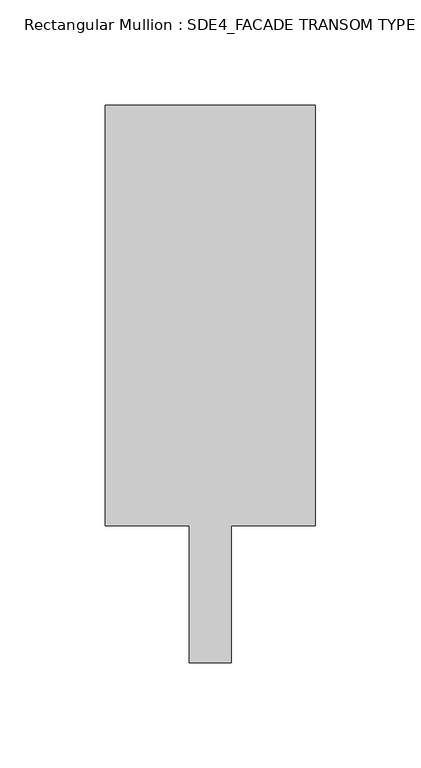
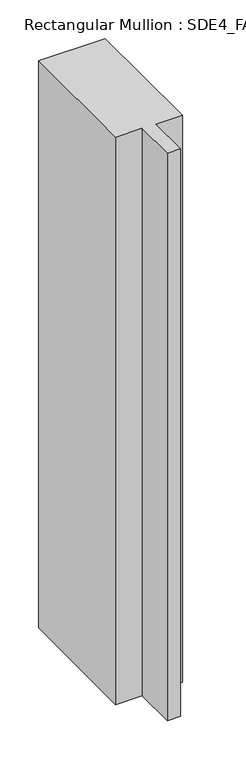
"""IFC4 building model written with IfcOpenShell, lengths in millimetres: member geometry, Rectangular Mullion : SDE4_FACADE TRANSOM TYPE 2."""

from ifc_helpers import new_model, si_unit, frame, origin, place, context, project, spatial, polyline, outline, extrude, source, transform, mapped, element, save


def rectangular_mullion_sde4_facade_transom_type_2_b79b8d73(model_context):
    return source(origin(), model_context, "Body", "SweptSolid", [
        extrude(outline(polyline([(50.0, 132.5), (50.0, -67.5), (10.0, -67.5), (10.0, -132.5), (-10.0, -132.5), (-10.0, -67.5), (-50.0, -67.5), (-50.0, 132.5), (50.0, 132.5)])), frame((0.0, 0.0, -897.5), z_axis=(0.0, 0.0, 1.0), x_axis=(1.0, 0.0, 0.0)), (0.0, 0.0, 1.0), 897.5),
    ])


if __name__ == "__main__":
    model = new_model("IFC4")
    model_context = context("Model", 3, world=origin())
    ifc_project = project(units=[si_unit("LENGTHUNIT", "METRE", prefix="MILLI")], contexts=[model_context])
    site = spatial("IfcSite", under=ifc_project)
    building = spatial("IfcBuilding", under=site)
    placement = place(None, origin())
    rectangular_mullion_sde4_facade_transom_type_2_shape = rectangular_mullion_sde4_facade_transom_type_2_b79b8d73(model_context)
    element("IfcMember", 1, ObjectType="Rectangular Mullion : SDE4_FACADE TRANSOM TYPE 2", at=placement, inside=building, context=model_context, shape_type="MappedRepresentation", body=[
        mapped(rectangular_mullion_sde4_facade_transom_type_2_shape, transform((0.0, 0.0, 0.0), x_axis=(1.0, 0.0, 0.0), y_axis=(0.0, 1.0, 0.0), z_axis=(0.0, 0.0, 1.0))),
    ])
    save(model, "model.ifc")

# Revit data of these elements
# Type "Rectangular Mullion : SDE4_FACADE TRANSOM TYPE 2"
#   built-in parameter 1007322 = 0.869423 (stored number, unit not read)
#   built-in parameter 1007321 = 0.164042 (stored number, unit not read)
#   built-in parameter 1007320 = 0.164042 (stored number, unit not read)
